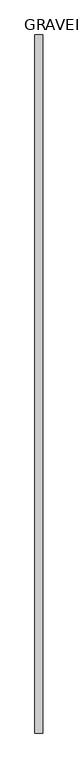
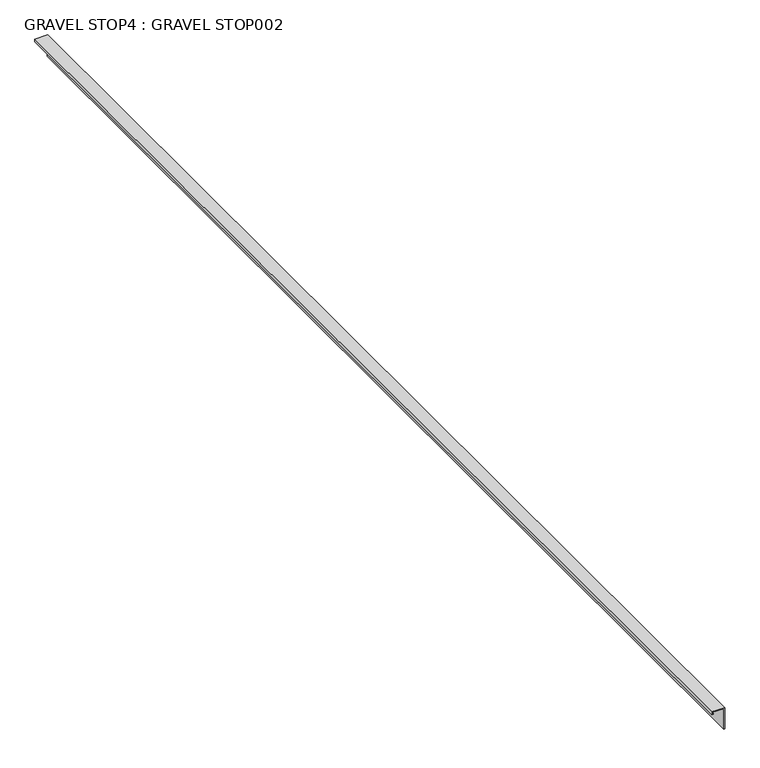
"""IFC4 building model written with IfcOpenShell, lengths in millimetres: proxy geometry, GRAVEL STOP4 : GRAVEL STOP002."""

import ifcopenshell
import ifcopenshell.guid

model = None  # the IFC model being written
_history = None  # IfcOwnerHistory: only IFC2X3 demands one
_inside = {}  # id of a spatial element -> (the spatial element, [elements in it])
_under = {}  # id of a project, library or spatial element -> (it, [spatial elements below it])
_declared = {}  # id of a project -> (the project, [libraries it declares])
_typed = {}  # id of a type object -> (the type object, [elements of that type])
_made_of = {}  # id of a material, layer set ... -> (it, [elements and type objects made of it])


def new_model(schema):
    """Start an empty IFC model of exactly this schema.

    Asked for "IFC4X3", IfcOpenShell would pick the latest addendum, in which some entities
    have other attributes; the version numbers below select the first issue.
    IFC2X3 requires an IfcOwnerHistory on every rooted entity: one is made here for all.
    """
    global model, _history
    if schema == "IFC4X3":
        model = ifcopenshell.file(schema_version=(4, 3, 0, 0))
    else:
        model = ifcopenshell.file(schema=schema)
    _inside.clear()
    _under.clear()
    _declared.clear()
    _typed.clear()
    _made_of.clear()
    _history = None
    if model.schema == "IFC2X3":
        org = make("IfcOrganization", Name="unknown")
        user = make(
            "IfcPersonAndOrganization",
            ThePerson=make("IfcPerson", FamilyName="unknown"),
            TheOrganization=org,
        )
        app = make(
            "IfcApplication",
            ApplicationDeveloper=org,
            Version="unknown",
            ApplicationFullName="unknown",
            ApplicationIdentifier="unknown",
        )
        _history = make(
            "IfcOwnerHistory",
            OwningUser=user,
            OwningApplication=app,
            ChangeAction="ADDED",
            CreationDate=0,
        )
    return model


def make(cls, **values):
    """One entity of the class cls with the attributes given. An attribute that is None is left unset."""
    return model.create_entity(
        cls, **{name: value for name, value in values.items() if value is not None}
    )


def rooted(cls, **values):
    """An entity with a GlobalId (a new one), such as an element, a storey or a relation."""
    return make(cls, GlobalId=ifcopenshell.guid.new(), OwnerHistory=_history, **values)


def si_unit(unit_type, name, prefix=None):
    """IfcSIUnit, for example si_unit("LENGTHUNIT", "METRE", prefix="MILLI")."""
    return make("IfcSIUnit", UnitType=unit_type, Prefix=prefix, Name=name)


def assignment(units):
    """IfcUnitAssignment: the units of a project."""
    return None if units is None else make("IfcUnitAssignment", Units=units)


def point(xyz):
    """IfcCartesianPoint."""
    return None if xyz is None else make("IfcCartesianPoint", Coordinates=xyz)


def direction(xyz):
    """IfcDirection."""
    return None if xyz is None else make("IfcDirection", DirectionRatios=xyz)


def frame(location, z_axis=None, x_axis=None):
    """IfcAxis2Placement3D, a coordinate frame: its origin and axes. An axis left out is left unset."""
    return make(
        "IfcAxis2Placement3D",
        Location=point(location),
        Axis=direction(z_axis),
        RefDirection=direction(x_axis),
    )


def origin():
    """The frame at (0, 0, 0) with its axes left unset."""
    return frame((0.0, 0.0, 0.0))


def place(relative_to, where):
    """IfcLocalPlacement: puts the frame where relative to a parent placement (None: the world)."""
    return make(
        "IfcLocalPlacement", PlacementRelTo=relative_to, RelativePlacement=where
    )


def context(
    kind, dimensions, precision=None, world=None, true_north=None, identifier=None
):
    """IfcGeometricRepresentationContext, for example the 3D "Model" context."""
    return make(
        "IfcGeometricRepresentationContext",
        ContextIdentifier=identifier,
        ContextType=kind,
        CoordinateSpaceDimension=dimensions,
        Precision=precision,
        WorldCoordinateSystem=world,
        TrueNorth=true_north,
    )


def project(units=None, contexts=None):
    """IfcProject with its units and contexts."""
    return rooted(
        "IfcProject",
        Name="project",
        RepresentationContexts=contexts,
        UnitsInContext=assignment(units),
    )


def spatial(cls, under=None, at=None, **own):
    """A site, building, storey or space (cls), placed at a placement, below another one or the project."""
    s = rooted(cls, ObjectPlacement=at, **own)
    if under is not None:
        _under.setdefault(under.id(), (under, []))[1].append(s)
    return s


def polyline(points):
    """IfcPolyline through the points."""
    return make("IfcPolyline", Points=[point(p) for p in points])


def outline(outer, holes=None, kind="AREA"):
    """IfcArbitraryClosedProfileDef: a profile drawn as a closed curve; with holes, ...WithVoids."""
    if holes is None:
        return make("IfcArbitraryClosedProfileDef", ProfileType=kind, OuterCurve=outer)
    return make(
        "IfcArbitraryProfileDefWithVoids",
        ProfileType=kind,
        OuterCurve=outer,
        InnerCurves=holes,
    )


def extrude(swept, where, along, depth):
    """IfcExtrudedAreaSolid: the profile swept, set in the frame where, extruded along a direction by depth."""
    return make(
        "IfcExtrudedAreaSolid",
        SweptArea=swept,
        Position=where,
        ExtrudedDirection=direction(along),
        Depth=depth,
    )


def shape(context_of_items, identifier, shape_type, items):
    """IfcShapeRepresentation: the items that make up one representation, for example the "Body"."""
    return make(
        "IfcShapeRepresentation",
        ContextOfItems=context_of_items,
        RepresentationIdentifier=identifier,
        RepresentationType=shape_type,
        Items=items,
    )


def source(mapping_origin, context_of_items, identifier, shape_type, items):
    """IfcRepresentationMap: a shape defined once, which mapped items show again and again."""
    return make(
        "IfcRepresentationMap",
        MappingOrigin=mapping_origin,
        MappedRepresentation=shape(context_of_items, identifier, shape_type, items),
    )


def transform(
    local_origin,
    x_axis=None,
    y_axis=None,
    z_axis=None,
    scale=None,
    scale2=None,
    scale3=None,
    uniform=True,
):
    """IfcCartesianTransformationOperator3D, or its non-uniform kind. x_axis, y_axis, z_axis: its Axis1, 2, 3."""
    if uniform:
        return make(
            "IfcCartesianTransformationOperator3D",
            Axis1=direction(x_axis),
            Axis2=direction(y_axis),
            LocalOrigin=point(local_origin),
            Scale=scale,
            Axis3=direction(z_axis),
        )
    return make(
        "IfcCartesianTransformationOperator3DnonUniform",
        Axis1=direction(x_axis),
        Axis2=direction(y_axis),
        LocalOrigin=point(local_origin),
        Scale=scale,
        Axis3=direction(z_axis),
        Scale2=scale2,
        Scale3=scale3,
    )


def mapped(mapping_source, mapping_target):
    """IfcMappedItem: shows the shape of a source again, moved by a transform."""
    return make(
        "IfcMappedItem", MappingSource=mapping_source, MappingTarget=mapping_target
    )


def made_of(thing, what):
    """Note that an element or type object is made of a material, layer set ...; save() writes the relation."""
    if what is not None:
        _made_of.setdefault(what.id(), (what, []))[1].append(thing)
    return thing


def element(
    cls,
    number,
    at=None,
    inside=None,
    cuts=None,
    type_object=None,
    material=None,
    context=None,
    identifier="Body",
    shape_type=None,
    held_by="IfcProductDefinitionShape",
    body=None,
    shapes=None,
    **own,
):
    """One element of the class cls, such as IfcWall. Its Tag is "e" and its number.

    at: its placement. inside: the storey or other place that contains it. cuts: it is an
    opening in that element (IfcRelVoidsElement). A single representation is given by context,
    identifier, shape_type and body (its items); several are given by shapes. held_by: the class
    of the entity that holds the representations. save() writes the other relations.
    """
    e = rooted(cls, Tag="e%d" % number, ObjectPlacement=at, **own)
    if body is not None:
        shapes = [shape(context, identifier, shape_type, body)]
    if shapes is not None:
        e.Representation = make(held_by, Representations=shapes)
    if inside is not None:
        _inside.setdefault(inside.id(), (inside, []))[1].append(e)
    if cuts is not None:
        rooted(
            "IfcRelVoidsElement", RelatingBuildingElement=cuts, RelatedOpeningElement=e
        )
    if type_object is not None:
        _typed.setdefault(type_object.id(), (type_object, []))[1].append(e)
    return made_of(e, material)


def aggregate(whole, parts):
    """IfcRelAggregates: a whole, such as a stair, and the parts it consists of."""
    return rooted("IfcRelAggregates", RelatingObject=whole, RelatedObjects=parts)


def save(model, path):
    """Write the relations noted so far, then the file.

    IfcRelAggregates (storeys below a building ...), IfcRelContainedInSpatialStructure (elements
    in a storey), IfcRelDefinesByType, IfcRelAssociatesMaterial and IfcRelDeclares: one each for
    every whole, place, type object, material and project.
    """
    for whole, parts in _under.values():
        aggregate(whole, parts)
    for where, things in _inside.values():
        rooted(
            "IfcRelContainedInSpatialStructure",
            RelatedElements=things,
            RelatingStructure=where,
        )
    for kind, things in _typed.values():
        rooted("IfcRelDefinesByType", RelatedObjects=things, RelatingType=kind)
    for what, things in _made_of.values():
        rooted("IfcRelAssociatesMaterial", RelatedObjects=things, RelatingMaterial=what)
    for by, libraries in _declared.values():
        rooted("IfcRelDeclares", RelatingContext=by, RelatedDefinitions=libraries)
    model.write(path)


def gravel_stop4_gravel_stop002_7d4a8986(model_context):
    return source(origin(), model_context, "Body", "SweptSolid", [
        extrude(outline(polyline([(40234.4061757, -2790.7286469), (40197.5761757, -2790.7286469), (40197.5761757, -2789.4586469), (40235.6761757, -2789.4586469), (40235.6761757, -2811.6836469), (40230.9263757, -2811.6836469), (40230.9263757, -2808.6811906), (40232.1963757, -2808.6811906), (40232.1963757, -2810.4136469), (40234.4061757, -2810.4136469), (40234.4061757, -2790.7286469)])), frame((0.0, 1000.0000001, 0.0), z_axis=(0.0, 1.0, 0.0), x_axis=(0.0, 0.0, 1.0)), (0.0, 0.0, 1.0), 2000.25),
    ])


if __name__ == "__main__":
    model = new_model("IFC4")
    model_context = context("Model", 3, world=origin())
    ifc_project = project(units=[si_unit("LENGTHUNIT", "METRE", prefix="MILLI")], contexts=[model_context])
    site = spatial("IfcSite", under=ifc_project)
    building = spatial("IfcBuilding", under=site)
    placement = place(None, origin())
    gravel_stop4_gravel_stop002_shape = gravel_stop4_gravel_stop002_7d4a8986(model_context)
    element("IfcBuildingElementProxy", 1, Name="GRAVEL STOP4 : GRAVEL STOP002", ObjectType="GRAVEL STOP4 : GRAVEL STOP002", at=placement, inside=building, context=model_context, shape_type="MappedRepresentation", body=[
        mapped(gravel_stop4_gravel_stop002_shape, transform((0.0, 0.0, 0.0), x_axis=(1.0, 0.0, 0.0), y_axis=(0.0, 1.0, 0.0), z_axis=(0.0, 0.0, 1.0))),
    ])
    save(model, "model.ifc")

# Revit data of these elements
# Type "GRAVEL STOP4 : GRAVEL STOP002"
#   NameOverride = "GRAVEL STOP002"
# Element 1 (IfcBuildingElementProxy, "GRAVEL STOP4 : GRAVEL STOP002")
#   Materials on its faces: "COPPER STUCCO J BEAD"
# Materials
#   "COPPER STUCCO J BEAD": class "Unassigned", colour RGB 251 232 155, transparency 0, Cost = 0
